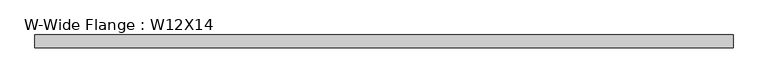
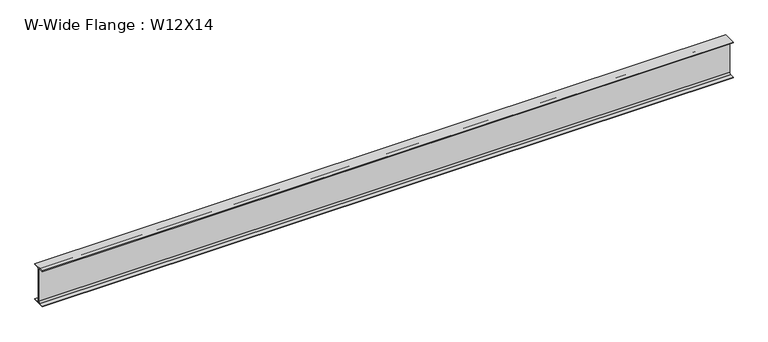
"""IFC4 building model written with IfcOpenShell, lengths in millimetres: beam geometry, W-Wide Flange : W12X14."""

from ifc_helpers import new_model, si_unit, point, frame, frame_2d, origin, place, context, project, spatial, polyline, circle_curve, trimmed, segment, composite_curve, outline, extrude, source, transform, mapped, element, save


def w_wide_flange_w12x14_8a244811(model_context):
    return source(origin(), model_context, "Body", "SweptSolid", [
        extrude(outline(composite_curve([segment(polyline([(-50.419, -145.415), (-15.875, -145.415)]), True, "CONTINUOUS"), segment(trimmed(circle_curve(frame_2d((-15.875, -132.08)), 13.335), [point((-15.875, -145.415))], [point((-2.54, -132.08))], True, "CARTESIAN"), True, "CONTINUOUS"), segment(polyline([(-2.54, -132.08), (-2.54, 132.08)]), True, "CONTINUOUS"), segment(trimmed(circle_curve(frame_2d((-15.875, 132.08)), 13.335), [point((-2.54, 132.08))], [point((-15.875, 145.415))], True, "CARTESIAN"), True, "CONTINUOUS"), segment(polyline([(-15.875, 145.415), (-50.419, 145.415), (-50.419, 151.13), (50.419, 151.13), (50.419, 145.415), (15.875, 145.415)]), True, "CONTINUOUS"), segment(trimmed(circle_curve(frame_2d((15.875, 132.08)), 13.335), [point((15.875, 145.415))], [point((2.54, 132.08))], True, "CARTESIAN"), True, "CONTINUOUS"), segment(polyline([(2.54, 132.08), (2.54, -132.08)]), True, "CONTINUOUS"), segment(trimmed(circle_curve(frame_2d((15.875, -132.08)), 13.335), [point((2.54, -132.08))], [point((15.875, -145.415))], True, "CARTESIAN"), True, "CONTINUOUS"), segment(polyline([(15.875, -145.415), (50.419, -145.415), (50.419, -151.13), (-50.419, -151.13), (-50.419, -145.415)]), True, "CONTINUOUS")], self_intersect=False)), frame((-2781.681, 0.0, 0.0), z_axis=(1.0, 0.0, 0.0), x_axis=(0.0, 1.0, 0.0)), (0.0, 0.0, 1.0), 5524.754),
    ])


if __name__ == "__main__":
    model = new_model("IFC4")
    model_context = context("Model", 3, world=origin())
    ifc_project = project(units=[si_unit("LENGTHUNIT", "METRE", prefix="MILLI")], contexts=[model_context])
    site = spatial("IfcSite", under=ifc_project)
    building = spatial("IfcBuilding", under=site)
    placement = place(None, origin())
    w_wide_flange_w12x14_shape = w_wide_flange_w12x14_8a244811(model_context)
    element("IfcBeam", 1, ObjectType="W-Wide Flange : W12X14", at=placement, inside=building, context=model_context, shape_type="MappedRepresentation", body=[
        mapped(w_wide_flange_w12x14_shape, transform((0.0, 0.0, 0.0), x_axis=(1.0, 0.0, 0.0), y_axis=(0.0, 1.0, 0.0), z_axis=(0.0, 0.0, 1.0))),
    ])
    save(model, "model.ifc")

# Revit data of these elements
# Type "W-Wide Flange : W12X14"
#   Assembly Code = "B10"
#   W = 14
#   Length [instance default] = 5' - 0"
#   bf = 0' - 3.97"
#   d = 0' - 11.9"
#   k = 0' - 0 3/4"
#   k2 = 0' - 0.525"
#   tf = 0' - 0.225"
#   tw = 0' - 0.2"
#   A = 0.0288889 SF
#   Structural Material [instance default] = Steel ASTM A992
# Element 1 (IfcBeam, "W-Wide Flange : W12X14")
#   Materials on its faces: "Steel ASTM A992"
# Materials
#   "Steel ASTM A992": class "Metal", colour RGB 199 199 199, transparency 0, Description = "Structural steel 50ksi", Cost = 0
